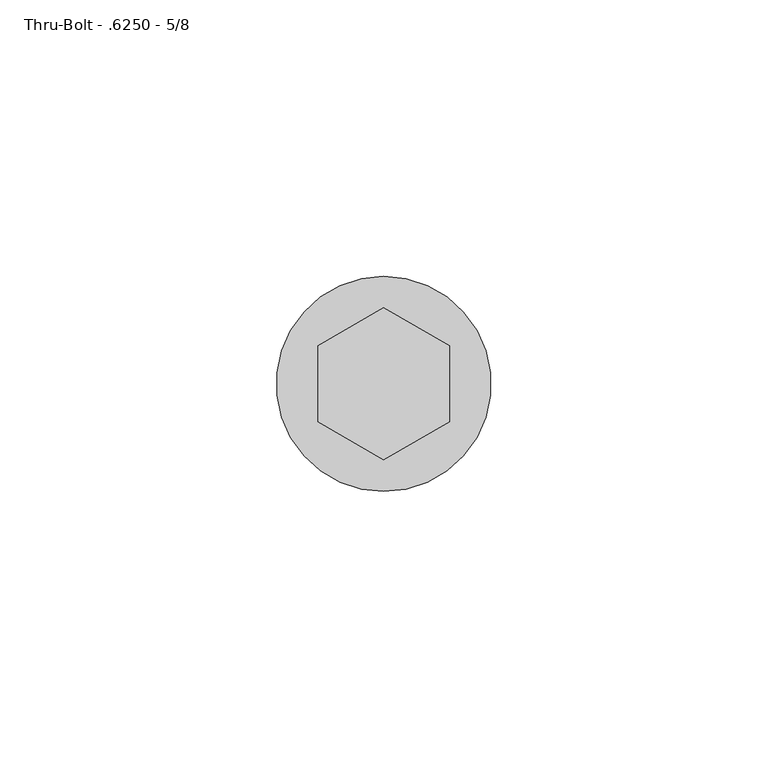
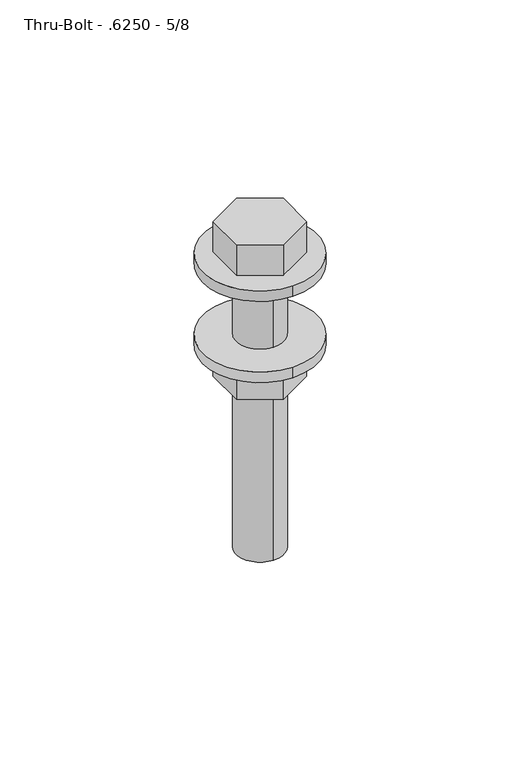
"""IFC4 building model written with IfcOpenShell, lengths in millimetres: fastener geometry, 060523 - W_P_C - Fastenings - Generic : Thru-Bolt - .6250 - 5/8."""

from ifc_helpers import new_model, si_unit, point, frame, origin, origin_with_axes, origin_2d, place, context, project, spatial, polyline, circle_curve, trimmed, segment, composite_curve, outline, extrude, source, transform, mapped, element, save


def thru_bolt_6250_5_8_6d7a9ef5(model_context):
    return source(origin(), model_context, "Body", "SweptSolid", [
        extrude(outline(composite_curve([segment(trimmed(circle_curve(origin_2d(), 19.446875), [point((0.0, 19.446875))], [point((0.0, -19.446875))], False, "CARTESIAN"), True, "CONTINUOUS"), segment(trimmed(circle_curve(origin_2d(), 19.446875), [point((0.0, -19.446875))], [point((0.0, 19.446875))], False, "CARTESIAN"), True, "CONTINUOUS")], self_intersect=False)), origin_with_axes(), (0.0, 0.0, 1.0), 3.7703125),
        extrude(outline(composite_curve([segment(trimmed(circle_curve(origin_2d(), 19.446875), [point((0.0, 19.446875))], [point((0.0, -19.446875))], False, "CARTESIAN"), True, "CONTINUOUS"), segment(trimmed(circle_curve(origin_2d(), 19.446875), [point((0.0, -19.446875))], [point((0.0, 19.446875))], False, "CARTESIAN"), True, "CONTINUOUS")], self_intersect=False)), frame((0.0, 0.0, -29.1703125), z_axis=(0.0, 0.0, 1.0), x_axis=(1.0, 0.0, 0.0)), (0.0, 0.0, 1.0), 3.7703125),
        extrude(outline(polyline([(-11.90625, -6.8740766), (-11.90625, 6.8740766), (0.0, 13.7481533), (11.90625, 6.8740766), (11.90625, -6.8740766), (0.0, -13.7481533), (-11.90625, -6.8740766)])), frame((0.0, 0.0, -40.48125), z_axis=(0.0, 0.0, 1.0), x_axis=(1.0, 0.0, 0.0)), (0.0, 0.0, 1.0), 11.3109375),
        extrude(outline(polyline([(-11.90625, 6.8740766), (0.0, 13.7481533), (11.90625, 6.8740766), (11.90625, -6.8740766), (0.0, -13.7481533), (-11.90625, -6.8740766), (-11.90625, 6.8740766)])), frame((0.0, 0.0, 3.7703125), z_axis=(0.0, 0.0, 1.0), x_axis=(1.0, 0.0, 0.0)), (0.0, 0.0, 1.0), 11.3109375),
        extrude(outline(composite_curve([segment(trimmed(circle_curve(origin_2d(), 8.1359375), [point((0.0, -8.1359375))], [point((0.0, 8.1359375))], False, "CARTESIAN"), True, "CONTINUOUS"), segment(trimmed(circle_curve(origin_2d(), 8.1359375), [point((0.0, 8.1359375))], [point((0.0, -8.1359375))], False, "CARTESIAN"), True, "CONTINUOUS")], self_intersect=False)), frame((0.0, 0.0, -101.6), z_axis=(0.0, 0.0, 1.0), x_axis=(1.0, 0.0, 0.0)), (0.0, 0.0, 1.0), 105.3703125),
    ])


if __name__ == "__main__":
    model = new_model("IFC4")
    model_context = context("Model", 3, world=origin())
    ifc_project = project(units=[si_unit("LENGTHUNIT", "METRE", prefix="MILLI")], contexts=[model_context])
    site = spatial("IfcSite", under=ifc_project)
    building = spatial("IfcBuilding", under=site)
    placement = place(None, origin())
    thru_bolt_6250_5_8_shape = thru_bolt_6250_5_8_6d7a9ef5(model_context)
    element("IfcFastener", 1, ObjectType="060523 - W_P_C - Fastenings - Generic : Thru-Bolt - .6250 - 5/8", at=placement, inside=building, context=model_context, shape_type="MappedRepresentation", body=[
        mapped(thru_bolt_6250_5_8_shape, transform((0.0, 0.0, 0.0), x_axis=(1.0, 0.0, 0.0), y_axis=(0.0, 1.0, 0.0), z_axis=(0.0, 0.0, 1.0))),
    ])
    save(model, "model.ifc")

# Revit data of these elements
# Type "060523 - W_P_C - Fastenings - Generic : Thru-Bolt - .6250 - 5/8"
#   Washer_Thickness = 0' - 0 19/128"
#   Washer Radius = 0' - 0 49/64"
#   Washer Offset - Head = 0' - 0 19/128"
#   Washer Offset = 0' - 0 19/128"
#   Thickness_of_Substrate [instance default] = 0' - 1"
#   Side = 0' - 0.54199"
#   Radius = 0' - 0 41/128"
#   Length [instance default] = 0' - 4"
#   Head Size = 0' - 0 15/16"
#   Head Radius = 0' - 0 15/32"
#   Head Height = 0' - 0 57/128"
#   Double Diameter = 0' - 1 9/32"
#   Diameter = 0' - 0 41/64"
#   Default Elevation = 4' - 0"
#   Washer_Nut_Visibility = yes
#   Washer_Head_Visibility = yes
#   Round_Head_Visibility = no
#   Point Visibility = no
#   Nut_Visibility = yes
#   Hex_Head_Visiblilty = yes
#   Washer Material = none
#   Bolt Material (Size) = AT SILL - FASTENER AT 24" O.C.
# Element 1 (IfcFastener, "060523 - W_P_C - Fastenings - Generic : Thru-Bolt - .6250 - 5/8")
#   Materials on its faces: "AT SILL - FASTENER AT 24\" O.C."
# Materials
#   "AT SILL - FASTENER AT 24\" O.C.": class "Generic", colour RGB 120 120 120, transparency 0, Cost = 0
